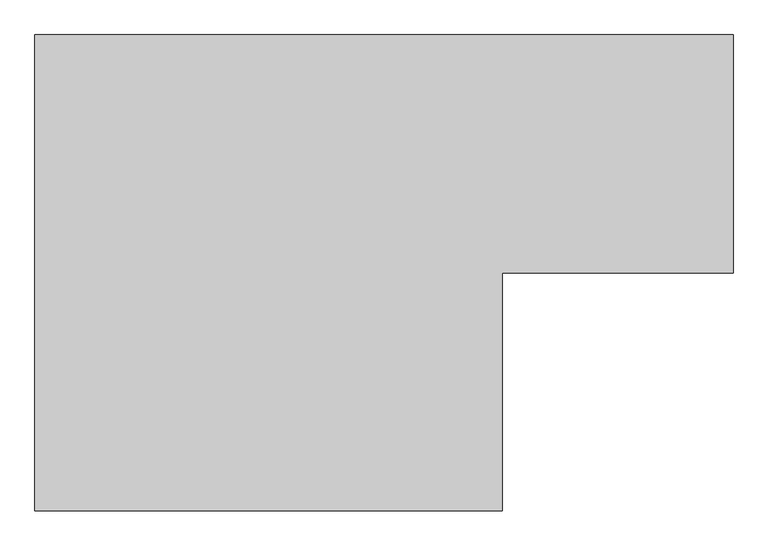
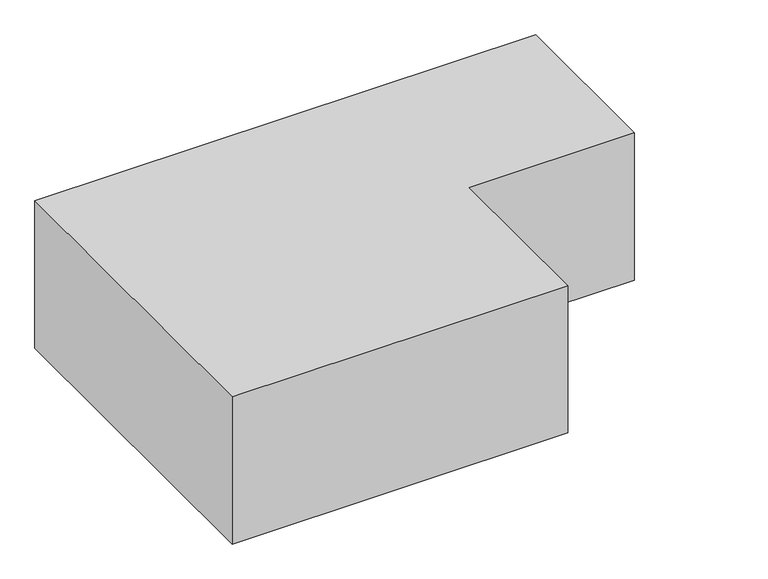
"""IFC4 building model written with IfcOpenShell, lengths in millimetres: proxy geometry, Приточная установка_П2 : СКВ ВОХ 13/10."""

from ifc_helpers import new_model, si_unit, origin, origin_with_axes, place, context, project, spatial, polyline, outline, extrude, source, transform, mapped, element, save


def mechanical_equipment_88f833ef(model_context):
    return source(origin(), model_context, "Body", "SweptSolid", [
        extrude(outline(polyline([(3957.5, 0.0), (3957.5, -1350.0), (2650.0, -1350.0), (2650.0, -2700.0), (0.0, -2700.0), (0.0, 0.0), (3957.5, 0.0)])), origin_with_axes(), (0.0, 0.0, 1.0), 1230.0),
    ])


if __name__ == "__main__":
    model = new_model("IFC4")
    model_context = context("Model", 3, world=origin())
    ifc_project = project(units=[si_unit("LENGTHUNIT", "METRE", prefix="MILLI")], contexts=[model_context])
    site = spatial("IfcSite", under=ifc_project)
    building = spatial("IfcBuilding", under=site)
    placement = place(None, origin())
    mechanical_equipment_shape = mechanical_equipment_88f833ef(model_context)
    element("IfcBuildingElementProxy", 1, Name="Приточная установка_П2 : СКВ ВОХ 13/10", ObjectType="Приточная установка_П2 : СКВ ВОХ 13/10", at=placement, inside=building, context=model_context, shape_type="MappedRepresentation", body=[
        mapped(mechanical_equipment_shape, transform((0.0, 0.0, 0.0), x_axis=(1.0, 0.0, 0.0), y_axis=(0.0, 1.0, 0.0), z_axis=(0.0, 0.0, 1.0))),
    ])
    save(model, "model.ifc")

# Revit data of these elements
# Type "Приточная установка_П2 : СКВ ВОХ 13/10"
#   ADSK_Позиция = "21"
#   ADSK_Наименование = "Установка приточная"
#   ADSK_Марка = "СКВ ВОХ 13/1О-S-35,TY 4862-001-22330703-2014 комплектация по обосновывающему документу 0092.020.013.Р4. 0004.653.0000.3502 .003-ОВ.ОЛ2 инв. №10041702, 0092.020.013.Р4. 0004.653.0000.3502 .003-ОВ.Н2 инв.№10041724"
#   ADSK_Код изделия = "4261597"
#   ADSK_Завод-изготовитель = "ООО \"АЭРО ИКСИА\", Россия, г. Брянск, ИНН 3257017280, КП П 5261 О 1001, aero@ixia.su"
#   ADSK_Единица измерения = "компл."
#   Ширина соединения = 900 mm
#   Ширина приточной части = 1350 mm
#   Ширина клапана = 1100 mm
#   Ширина = 3957.5 mm
#   Подключение к теплосети = 80 mm
#   Длина = 2700 mm
#   Высота соединения = 1200 mm
#   Высота клапана = 1100 mm
#   Высота = 1230 mm
#   ADSK_Масса = 1295
#   ADSK_Количество = 1
#   Default Elevation = 0
